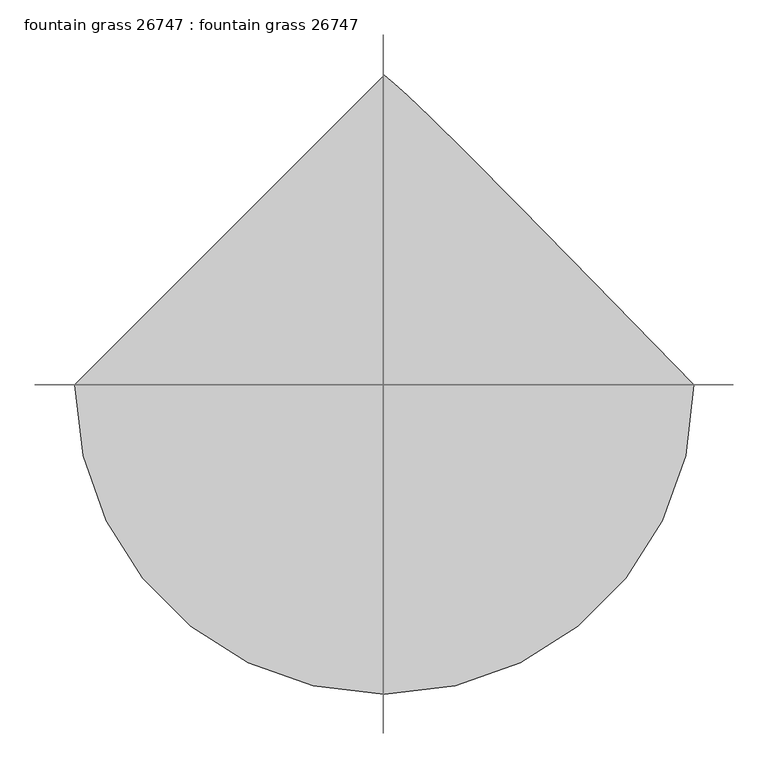
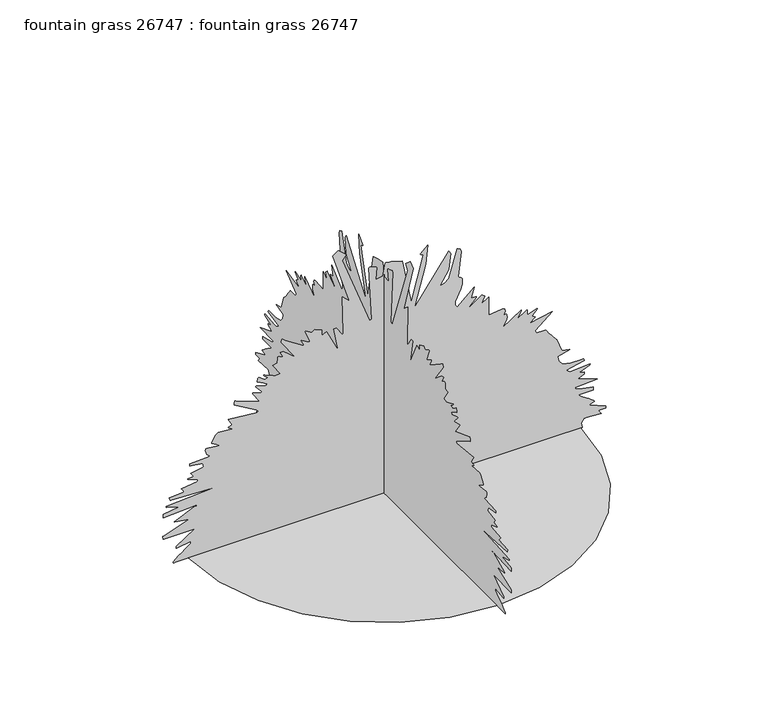
"""IFC4 building model written with IfcOpenShell, lengths in millimetres: proxy geometry, fountain grass 26747 : fountain grass 26747."""

import ifcopenshell
import ifcopenshell.guid

model = None  # the IFC model being written
_history = None  # IfcOwnerHistory: only IFC2X3 demands one
_inside = {}  # id of a spatial element -> (the spatial element, [elements in it])
_under = {}  # id of a project, library or spatial element -> (it, [spatial elements below it])
_declared = {}  # id of a project -> (the project, [libraries it declares])
_typed = {}  # id of a type object -> (the type object, [elements of that type])
_made_of = {}  # id of a material, layer set ... -> (it, [elements and type objects made of it])


def new_model(schema):
    """Start an empty IFC model of exactly this schema.

    Asked for "IFC4X3", IfcOpenShell would pick the latest addendum, in which some entities
    have other attributes; the version numbers below select the first issue.
    IFC2X3 requires an IfcOwnerHistory on every rooted entity: one is made here for all.
    """
    global model, _history
    if schema == "IFC4X3":
        model = ifcopenshell.file(schema_version=(4, 3, 0, 0))
    else:
        model = ifcopenshell.file(schema=schema)
    _inside.clear()
    _under.clear()
    _declared.clear()
    _typed.clear()
    _made_of.clear()
    _history = None
    if model.schema == "IFC2X3":
        org = make("IfcOrganization", Name="unknown")
        user = make(
            "IfcPersonAndOrganization",
            ThePerson=make("IfcPerson", FamilyName="unknown"),
            TheOrganization=org,
        )
        app = make(
            "IfcApplication",
            ApplicationDeveloper=org,
            Version="unknown",
            ApplicationFullName="unknown",
            ApplicationIdentifier="unknown",
        )
        _history = make(
            "IfcOwnerHistory",
            OwningUser=user,
            OwningApplication=app,
            ChangeAction="ADDED",
            CreationDate=0,
        )
    return model


def make(cls, **values):
    """One entity of the class cls with the attributes given. An attribute that is None is left unset."""
    return model.create_entity(
        cls, **{name: value for name, value in values.items() if value is not None}
    )


def rooted(cls, **values):
    """An entity with a GlobalId (a new one), such as an element, a storey or a relation."""
    return make(cls, GlobalId=ifcopenshell.guid.new(), OwnerHistory=_history, **values)


def si_unit(unit_type, name, prefix=None):
    """IfcSIUnit, for example si_unit("LENGTHUNIT", "METRE", prefix="MILLI")."""
    return make("IfcSIUnit", UnitType=unit_type, Prefix=prefix, Name=name)


def assignment(units):
    """IfcUnitAssignment: the units of a project."""
    return None if units is None else make("IfcUnitAssignment", Units=units)


def point(xyz):
    """IfcCartesianPoint."""
    return None if xyz is None else make("IfcCartesianPoint", Coordinates=xyz)


def direction(xyz):
    """IfcDirection."""
    return None if xyz is None else make("IfcDirection", DirectionRatios=xyz)


def frame(location, z_axis=None, x_axis=None):
    """IfcAxis2Placement3D, a coordinate frame: its origin and axes. An axis left out is left unset."""
    return make(
        "IfcAxis2Placement3D",
        Location=point(location),
        Axis=direction(z_axis),
        RefDirection=direction(x_axis),
    )


def origin():
    """The frame at (0, 0, 0) with its axes left unset."""
    return frame((0.0, 0.0, 0.0))


def place(relative_to, where):
    """IfcLocalPlacement: puts the frame where relative to a parent placement (None: the world)."""
    return make(
        "IfcLocalPlacement", PlacementRelTo=relative_to, RelativePlacement=where
    )


def context(
    kind, dimensions, precision=None, world=None, true_north=None, identifier=None
):
    """IfcGeometricRepresentationContext, for example the 3D "Model" context."""
    return make(
        "IfcGeometricRepresentationContext",
        ContextIdentifier=identifier,
        ContextType=kind,
        CoordinateSpaceDimension=dimensions,
        Precision=precision,
        WorldCoordinateSystem=world,
        TrueNorth=true_north,
    )


def project(units=None, contexts=None):
    """IfcProject with its units and contexts."""
    return rooted(
        "IfcProject",
        Name="project",
        RepresentationContexts=contexts,
        UnitsInContext=assignment(units),
    )


def spatial(cls, under=None, at=None, **own):
    """A site, building, storey or space (cls), placed at a placement, below another one or the project."""
    s = rooted(cls, ObjectPlacement=at, **own)
    if under is not None:
        _under.setdefault(under.id(), (under, []))[1].append(s)
    return s


def point_list(points):
    """IfcCartesianPointList2D or 3D."""
    cls = (
        "IfcCartesianPointList2D" if len(points[0]) == 2 else "IfcCartesianPointList3D"
    )
    return make(cls, CoordList=points)


def triangles(points, corners, closed=None, point_numbers=None):
    """IfcTriangulatedFaceSet: each triangle names its three corners, points numbered from 1."""
    return make(
        "IfcTriangulatedFaceSet",
        Coordinates=point_list(points),
        Closed=closed,
        CoordIndex=corners,
        PnIndex=point_numbers,
    )


def shape(context_of_items, identifier, shape_type, items):
    """IfcShapeRepresentation: the items that make up one representation, for example the "Body"."""
    return make(
        "IfcShapeRepresentation",
        ContextOfItems=context_of_items,
        RepresentationIdentifier=identifier,
        RepresentationType=shape_type,
        Items=items,
    )


def source(mapping_origin, context_of_items, identifier, shape_type, items):
    """IfcRepresentationMap: a shape defined once, which mapped items show again and again."""
    return make(
        "IfcRepresentationMap",
        MappingOrigin=mapping_origin,
        MappedRepresentation=shape(context_of_items, identifier, shape_type, items),
    )


def transform(
    local_origin,
    x_axis=None,
    y_axis=None,
    z_axis=None,
    scale=None,
    scale2=None,
    scale3=None,
    uniform=True,
):
    """IfcCartesianTransformationOperator3D, or its non-uniform kind. x_axis, y_axis, z_axis: its Axis1, 2, 3."""
    if uniform:
        return make(
            "IfcCartesianTransformationOperator3D",
            Axis1=direction(x_axis),
            Axis2=direction(y_axis),
            LocalOrigin=point(local_origin),
            Scale=scale,
            Axis3=direction(z_axis),
        )
    return make(
        "IfcCartesianTransformationOperator3DnonUniform",
        Axis1=direction(x_axis),
        Axis2=direction(y_axis),
        LocalOrigin=point(local_origin),
        Scale=scale,
        Axis3=direction(z_axis),
        Scale2=scale2,
        Scale3=scale3,
    )


def mapped(mapping_source, mapping_target):
    """IfcMappedItem: shows the shape of a source again, moved by a transform."""
    return make(
        "IfcMappedItem", MappingSource=mapping_source, MappingTarget=mapping_target
    )


def made_of(thing, what):
    """Note that an element or type object is made of a material, layer set ...; save() writes the relation."""
    if what is not None:
        _made_of.setdefault(what.id(), (what, []))[1].append(thing)
    return thing


def element(
    cls,
    number,
    at=None,
    inside=None,
    cuts=None,
    type_object=None,
    material=None,
    context=None,
    identifier="Body",
    shape_type=None,
    held_by="IfcProductDefinitionShape",
    body=None,
    shapes=None,
    **own,
):
    """One element of the class cls, such as IfcWall. Its Tag is "e" and its number.

    at: its placement. inside: the storey or other place that contains it. cuts: it is an
    opening in that element (IfcRelVoidsElement). A single representation is given by context,
    identifier, shape_type and body (its items); several are given by shapes. held_by: the class
    of the entity that holds the representations. save() writes the other relations.
    """
    e = rooted(cls, Tag="e%d" % number, ObjectPlacement=at, **own)
    if body is not None:
        shapes = [shape(context, identifier, shape_type, body)]
    if shapes is not None:
        e.Representation = make(held_by, Representations=shapes)
    if inside is not None:
        _inside.setdefault(inside.id(), (inside, []))[1].append(e)
    if cuts is not None:
        rooted(
            "IfcRelVoidsElement", RelatingBuildingElement=cuts, RelatedOpeningElement=e
        )
    if type_object is not None:
        _typed.setdefault(type_object.id(), (type_object, []))[1].append(e)
    return made_of(e, material)


def aggregate(whole, parts):
    """IfcRelAggregates: a whole, such as a stair, and the parts it consists of."""
    return rooted("IfcRelAggregates", RelatingObject=whole, RelatedObjects=parts)


def save(model, path):
    """Write the relations noted so far, then the file.

    IfcRelAggregates (storeys below a building ...), IfcRelContainedInSpatialStructure (elements
    in a storey), IfcRelDefinesByType, IfcRelAssociatesMaterial and IfcRelDeclares: one each for
    every whole, place, type object, material and project.
    """
    for whole, parts in _under.values():
        aggregate(whole, parts)
    for where, things in _inside.values():
        rooted(
            "IfcRelContainedInSpatialStructure",
            RelatedElements=things,
            RelatingStructure=where,
        )
    for kind, things in _typed.values():
        rooted("IfcRelDefinesByType", RelatedObjects=things, RelatingType=kind)
    for what, things in _made_of.values():
        rooted("IfcRelAssociatesMaterial", RelatedObjects=things, RelatingMaterial=what)
    for by, libraries in _declared.values():
        rooted("IfcRelDeclares", RelatingContext=by, RelatedDefinitions=libraries)
    model.write(path)


def fountain_grass_26747_fountain_grass_26747_87ae7408(model_context):
    return source(origin(), model_context, "Body", "Tessellation", [
        triangles([(-987.0455658, 0.0, 0.0001807), (-960.952173, -226.1654466, 0.0001807), (-886.6343983, -433.862035, 0.0001807), (-770.0484913, -617.1406734, 0.0001807), (-617.1406734, -770.0484913, 0.0001807), (-433.862035, -886.6343983, 0.0001807), (-226.1654466, -960.952173, 0.0001807), (4.31e-05, -987.0455658, 0.0001807), (226.1657009, -960.952173, 0.0001807), (433.862035, -886.6343983, 0.0001807), (617.1406734, -770.0484913, 0.0001807), (770.0484913, -617.1406734, 0.0001807), (886.6343983, -433.862035, 0.0001807), (960.952173, -226.1654466, 0.0001807), (987.0455658, 8.63e-05, 0.0001807), (666.2769184, 329.0287173, 0.0001807), (428.4772619, 571.2784656, 0.0001807), (259.8137924, 741.2118793, 0.0001807), (146.4631077, 853.2918114, 0.0001807), (74.5956602, 921.9810053, 0.0001807), (30.3837036, 961.7446392, 0.0001807), (-0.0001294, 987.0455658, 0.0001807), (-192.732222, -8.8e-06, 1335.7745705), (-213.2038286, -7.2e-06, 1310.1839813), (-75.0206025, 1.47e-05, 941.6939009), (-74.0421966, 1.47e-05, 941.9784039), (-72.5994794, 1.47e-05, 942.7098999), (-70.8743122, 1.46e-05, 943.7080948), (-69.0480519, 1.45e-05, 944.7977812), (-67.3038361, 1.45e-05, 945.7985195), (-65.8220043, 1.44e-05, 946.5300882), (-64.7846675, 1.44e-05, 946.8119751), (-80.1384406, -2.1e-06, 1223.1789722), (-79.3512975, -2.1e-06, 1223.3695129), (-78.4244554, -2.1e-06, 1223.8850338), (-77.4526488, -2.1e-06, 1224.6394936), (-76.5311389, -2.2e-06, 1225.5436535), (-75.2199908, -2.3e-06, 1227.4587982), (-75.0206025, -2.4e-06, 1228.2971191), (-39.1952093, -1.4e-06, 1212.9427511), (-44.3130519, 2.2e-06, 1151.5281858), (-8.4877319, 1.9e-06, 1156.6462601), (4.7327266, -1.8e-06, 1221.0427654), (6.8660195, -2.1e-06, 1223.1789722), (43.5436857, -1.6e-06, 1215.9958351), (88.7523407, -8e-07, 1202.7066027), (134.8136643, 1.32e-05, 967.2843447), (196.2285203, -5e-07, 1197.5909992), (183.550624, -1e-06, 1203.2526449), (181.3428736, -1.1e-06, 1205.4269308), (180.8747518, -1.1e-06, 1207.8246769), (216.700145, -3.3e-06, 1243.6512691), (206.4644507, 2.5e-06, 1146.4100389), (150.1674419, 1.53e-05, 931.4576797), (324.1773419, -3.2e-06, 1172.2011972), (334.4109833, -2.3e-06, 1156.8469019), (324.1773419, 2.6e-06, 1074.959967), (278.1144741, 6.8e-06, 1003.3091806), (303.186799, 6.4e-06, 1010.2737991), (322.3333048, 5.3e-06, 1028.8183794), (365.1195376, -3.2e-06, 1172.2011972), (380.7405318, -2.8e-06, 1165.3635332), (386.8136713, -1.8e-06, 1149.1050053), (371.0377447, 5.8e-06, 1020.4236883), (372.5033166, 6e-06, 1017.0835579), (375.3150999, 6.2e-06, 1014.6375589), (378.9295232, 6.3e-06, 1012.7299719), (382.8157322, 6.4e-06, 1011.0028244), (386.4301191, 6.5e-06, 1009.0952374), (389.2419024, 6.6e-06, 1006.6492384), (390.7100178, 6.8e-06, 1003.3091806), (390.8116467, 8.5e-06, 974.9780611), (383.7479064, 1e-05, 950.4898756), (355.0433722, 1.34e-05, 892.7557543), (354.7944775, 1.44e-05, 876.299128), (365.1195376, 1.54e-05, 860.0101513), (452.1246194, 1.08e-05, 936.7764685), (436.7703604, 1.39e-05, 885.5980516), (437.4358357, 1.38e-05, 884.2035873), (460.8495229, 1.41e-05, 882.1284233), (462.3608042, 1.42e-05, 880.4799774), (460.8800079, 1.46e-05, 876.8274387), (425.4318083, 1.61e-05, 841.6561117), (426.5341393, 1.66e-05, 839.537709), (430.7911832, 1.6e-05, 840.3353348), (487.9487409, 1.42e-05, 880.4799774), (489.1120783, 1.43e-05, 881.361319), (491.0831062, 1.43e-05, 880.6425402), (503.3030362, 1.48e-05, 870.2437563), (487.9487409, 1.69e-05, 834.4196348), (523.7754058, 1.54e-05, 860.0101513), (523.7754058, 2.12e-05, 762.7688484), (593.7116893, 2.08e-05, 769.8782982), (604.2222033, 2.1e-05, 765.8219324), (607.2778307, 2.16e-05, 755.5679798), (600.5443027, 2.27e-05, 737.1784046), (610.7779804, 2.27e-05, 737.1784046), (611.8422323, 2.27e-05, 736.5230667), (614.1129513, 2.29e-05, 734.0897123), (616.2186367, 2.32e-05, 729.1722799), (616.7773962, 2.37e-05, 721.0722656), (614.4152584, 2.44e-05, 709.086006), (595.4261922, 2.67e-05, 670.6456924), (687.546841, 2.3e-05, 732.0602577), (687.8186268, 2.35e-05, 728.1842588), (667.0770149, 2.55e-05, 691.118062), (716.0887762, 2.38e-05, 722.0933516), (718.2554317, 2.36e-05, 721.8266527), (719.3450455, 2.39e-05, 719.0986942), (717.5061316, 2.5e-05, 697.6534916), (718.2554317, 2.51e-05, 696.2361362), (720.4347319, 2.49e-05, 695.6976517), (766.5382404, 2.45e-05, 712.7029364), (769.4337759, 2.42e-05, 711.5904316), (768.6387663, 2.44e-05, 709.4415802), (744.2522461, 2.59e-05, 683.2440514), (743.8433321, 2.61e-05, 680.8819136), (759.1976274, 2.67e-05, 670.6456924), (728.4915802, 2.82e-05, 645.0577194), (845.0825741, 2.67e-05, 669.6881201), (759.1976274, 3.09e-05, 598.994906), (764.3157017, 3.19e-05, 583.6431541), (810.3760443, 3.19e-05, 583.6431541), (812.6900019, 3.21e-05, 579.4623047), (818.8519804, 3.26e-05, 570.8923699), (827.7013676, 3.33e-05, 559.353176), (838.0696301, 3.41e-05, 546.269636), (848.7985537, 3.49e-05, 533.064192), (858.7223665, 3.56e-05, 521.1643006), (866.6750788, 3.61e-05, 511.9923677), (892.2629791, 4.01e-05, 445.4596919), (933.2077909, 4.07e-05, 435.2234708), (871.793153, 4.16e-05, 419.8692118), (876.9112272, 4.31e-05, 394.2787316), (879.8754358, 4.33e-05, 391.6269676), (882.8904408, 4.35e-05, 388.2919604), (885.7733316, 4.37e-05, 384.6267408), (888.3361839, 4.39e-05, 380.9920063), (890.3960873, 4.41e-05, 377.7407876), (891.7651897, 4.43e-05, 375.2261882), (892.2629791, 4.44e-05, 373.8088692), (895.890156, 4.44e-05, 372.7801892), (938.3258652, 4.5e-05, 363.5726844), (999.7404305, 4.5e-05, 363.5726844), (1000.5278824, 4.5e-05, 362.5440044), (1001.4549334, 4.51e-05, 361.080976), (1002.425223, 4.52e-05, 359.3588428), (1003.3472597, 4.53e-05, 357.5503776), (1004.1219217, 4.54e-05, 355.8282443), (1004.6578629, 4.55e-05, 354.3652159), (1004.8585773, 4.56e-05, 353.3364996), (912.7354214, 4.68e-05, 332.86413), (913.6015022, 4.69e-05, 331.6373154), (915.8976557, 4.7e-05, 329.6383458), (919.1819029, 4.71e-05, 327.1415142), (923.0020912, 4.73e-05, 324.4110123), (926.9110823, 4.75e-05, 321.7160823), (930.4620283, 4.76e-05, 319.3259302), (933.2077909, 4.77e-05, 317.5123781), (949.6695042, 4.77e-05, 318.6757155), (1032.0797356, 4.76e-05, 324.6954789), (1035.5645519, 4.74e-05, 322.6279452), (1033.032221, 4.76e-05, 319.7526484), (979.2680609, 4.89e-05, 297.0400085), (1004.8585773, 4.92e-05, 291.9219162), (1004.8585773, 4.99e-05, 281.6857132), (975.3971489, 5.07e-05, 267.6446189), (974.1499866, 5.08e-05, 266.331436), (1071.3912169, 5.29e-05, 230.5068058), (958.7956913, 5.32e-05, 225.3889678), (958.7956913, 5.35e-05, 220.2708572), (979.2680609, 5.41e-05, 210.0351811), (1050.9188473, 5.5e-05, 194.6814126), (1050.9188473, 5.6e-05, 179.327626), (974.1499866, 5.6e-05, 179.327626), (978.767728, 5.62e-05, 175.5818881), (990.6523224, 5.67e-05, 167.0838239), (1006.8625975, 5.74e-05, 155.6789786), (1024.4520761, 5.81e-05, 143.2134423), (1051.9830992, 5.94e-05, 122.4842661), (1056.0369942, 5.96e-05, 117.9127791), (1055.1428627, 5.97e-05, 116.2480642), (1031.9527084, 6.02e-05, 108.5996212), (1030.4464777, 6.02e-05, 107.6770939), (1112.3334852, 6.24e-05, 71.8517007), (1112.3334852, 6.3e-05, 61.6157658), (1076.5093637, 6.3e-05, 61.6157658), (1088.8461107, 6.4e-05, 43.7974311), (1091.8611156, 6.42e-05, 41.1441501), (1004.8585773, 6.39e-05, 46.2622425), (989.504282, 6.51e-05, 25.7906269), (994.6223562, 6.66e-05, 0.2009925), (-1062.775609, 7.09e-05, 6.89e-05), (-1062.775609, 7.05e-05, 5.1179681), (-1049.4888474, 6.99e-05, 15.7529118), (-1033.944084, 6.92e-05, 27.9602914), (-1017.6728388, 6.84e-05, 40.5703616), (-1002.191589, 6.77e-05, 52.4138656), (-989.0343979, 6.71e-05, 62.3213777), (-979.7176701, 6.67e-05, 69.1234924), (-975.7730707, 6.66e-05, 71.6507864), (-975.7730707, 6.6e-05, 81.8864716), (-1047.4213137, 6.66e-05, 71.6507864), (-1047.4213137, 6.6e-05, 81.8864716), (-955.3006285, 6.23e-05, 143.3013185), (-1113.9564966, 6.23e-05, 143.3013185), (-1114.0479881, 6.22e-05, 144.6553964), (-1114.2638906, 6.21e-05, 147.0447673), (-1114.5102419, 6.19e-05, 150.0158069), (-1114.6931522, 6.17e-05, 153.1156177), (-1114.7261444, 6.16e-05, 155.891066), (-1114.5102419, 6.14e-05, 157.8885276), (-1113.9564966, 6.14e-05, 158.6551051), (-986.0066757, 5.87e-05, 204.7161744), (-1054.7643974, 5.81e-05, 213.3275311), (-1057.6574621, 5.8e-05, 214.9521049), (-955.3006285, 5.53e-05, 261.0126836), (-945.06448, 5.53e-05, 261.0126836), (-945.06448, 5.5e-05, 266.130776), (-1113.9564966, 5.56e-05, 255.8945912), (-1113.9564966, 5.44e-05, 276.3669608), (-1032.0695618, 5.38e-05, 286.6031456), (-1098.6022739, 5.26e-05, 307.0755152), (-1098.6022739, 5.22e-05, 312.1910823), (-852.941324, 5.13e-05, 327.5453776), (-1078.1298317, 5.07e-05, 337.7815624), (-1082.9660191, 4.99e-05, 351.3121319), (-1083.2479786, 4.98e-05, 353.1358578), (-1006.4790453, 4.95e-05, 358.253932), (-1021.1679016, 4.84e-05, 377.3064754), (-1021.8333406, 4.83e-05, 378.7237945), (-939.9464058, 4.77e-05, 388.9599792), (-939.9464058, 4.71e-05, 399.196164), (-983.6648129, 4.62e-05, 414.4208888), (-989.0952953, 4.6e-05, 417.5603411), (-991.1248226, 4.58e-05, 419.6685336), (-960.4187754, 4.55e-05, 424.7866442), (-975.1050156, 4.44e-05, 443.8391513), (-975.7730707, 4.43e-05, 445.2590137), (-909.2403585, 4.37e-05, 455.4926551), (-914.3558893, 4.25e-05, 475.965061), (-980.8911449, 4.19e-05, 486.2012458), (-980.8911449, 4.13e-05, 496.4374306), (-878.5317678, 4.1e-05, 501.5555048), (-879.1134184, 4.09e-05, 503.3716003), (-888.6028828, 4.02e-05, 513.6840159), (-893.8860632, 4e-05, 516.9098001), (-900.7211838, 3.88e-05, 540.5851356), (-900.558621, 3.85e-05, 544.4840255), (-899.0041374, 3.82e-05, 547.6158474), (-894.7090508, 3.84e-05, 548.9721963), (-839.7257063, 3.85e-05, 543.0539892), (-832.4714979, 3.85e-05, 542.4977368), (-834.0945093, 3.85e-05, 545.8555987), (-865.9461262, 3.72e-05, 565.5888419), (-868.2956194, 3.7e-05, 568.088217), (-868.4048424, 3.65e-05, 572.164894), (-848.5039495, 3.46e-05, 604.96896), (-842.4562082, 3.44e-05, 611.1792641), (-837.5895721, 3.42e-05, 614.1485596), (-765.9387857, 3.46e-05, 609.030449), (-780.5183464, 3.41e-05, 617.4352776), (-785.6364206, 3.37e-05, 622.5609821), (-786.4086119, 3.36e-05, 624.384708), (-767.3586119, 3.34e-05, 628.6646067), (-765.9387857, 3.33e-05, 629.5027822), (-786.4086119, 3.12e-05, 665.3269037), (-637.9889648, 3.21e-05, 649.9752245), (-637.7984241, 3.21e-05, 650.9530718), (-637.2828306, 3.2e-05, 652.395789), (-636.5284435, 3.19e-05, 654.1204657), (-635.6242109, 3.18e-05, 655.946735), (-634.6564648, 3.17e-05, 657.6916866), (-633.7090662, 3.16e-05, 659.1725555), (-632.8733614, 3.15e-05, 660.2088295), (-755.7025646, 2.72e-05, 731.8596159), (-755.710195, 2.71e-05, 734.6180958), (-755.6593987, 2.69e-05, 738.1944036), (-755.4384092, 2.67e-05, 742.1339161), (-754.9329895, 2.65e-05, 745.9743793), (-754.0313004, 2.63e-05, 749.26117), (-752.6190319, 2.61e-05, 751.5344324), (-750.5844904, 2.6e-05, 752.3319855), (-627.7552872, 2.88e-05, 706.2717155), (-663.6860882, 2.56e-05, 759.6675116), (-663.5794086, 2.54e-05, 762.5682066), (-660.4755283, 2.56e-05, 763.5054314), (-620.4934484, 2.58e-05, 751.3083561), (-617.5191387, 2.6e-05, 752.3319855), (-618.27854, 2.56e-05, 755.4434961), (-647.6638103, 2.37e-05, 790.1982788), (-648.2251133, 2.36e-05, 793.2742538), (-645.0653498, 2.38e-05, 794.1149729), (-597.0467328, 2.45e-05, 777.9225019), (-596.4675894, 2.44e-05, 778.9130665), (-595.0452198, 2.43e-05, 780.3888485), (-593.2570295, 2.42e-05, 782.1490608), (-591.5755551, 2.41e-05, 784.0032354), (-590.4782747, 2.4e-05, 785.7507305), (-590.4376522, 2.39e-05, 787.201078), (-591.9286222, 2.39e-05, 788.1586504), (-637.9889648, 2.24e-05, 813.7466234), (-639.6145197, 2.21e-05, 815.2045286), (-640.0666723, 2.19e-05, 818.265243), (-638.3851616, 2.15e-05, 826.5253492), (-636.7163681, 2.14e-05, 830.3861601), (-634.8012234, 2.12e-05, 833.1724726), (-632.8733614, 2.11e-05, 834.218993), (-630.4730719, 2.12e-05, 834.2443548), (-602.164807, 2.24e-05, 813.7466234), (-586.810548, 2.2e-05, 818.8646976), (-606.0256179, 2.11e-05, 834.9200403), (-607.7909171, 2.1e-05, 837.6987951), (-607.2829176, 2.08e-05, 839.3370672), (-603.6684943, 2.09e-05, 838.9128925), (-561.8702826, 2.2e-05, 820.0915123), (-550.9864265, 2.24e-05, 813.7466234), (-525.3959464, 2.2e-05, 818.8646976), (-559.8662261, 1.89e-05, 871.7906096), (-561.2226113, 1.87e-05, 875.1611887), (-540.7502054, 1.84e-05, 880.2793356), (-537.9714506, 1.73e-05, 906.7536644), (-536.9859366, 1.7e-05, 909.870262), (-535.6321312, 1.66e-05, 910.9878536), (-533.2191244, 1.68e-05, 912.2654646), (-529.3558064, 1.69e-05, 911.5212513), (-510.0416511, 1.72e-05, 900.7517052), (-525.3959464, 1.53e-05, 931.4576797), (-510.0416511, 1.53e-05, 931.4576797), (-448.6270494, 1.84e-05, 880.2793356), (-520.2778358, 1.23e-05, 982.63864), (-520.4962818, 1.22e-05, 984.7163475), (-516.051277, 1.16e-05, 996.9642191), (-515.2257823, 1.15e-05, 998.3459661), (-515.1597616, 1.14e-05, 997.9903919), (-498.3728866, 1.21e-05, 985.7882298), (-408.0734565, 1.55e-05, 927.9093498), (-402.5667432, 1.56e-05, 926.342149), (-417.4790597, 1.45e-05, 951.9148613), (-418.5687098, 1.42e-05, 955.282897), (-417.9210385, 1.38e-05, 957.0481962), (-415.5080317, 1.41e-05, 957.1853245), (-380.6389392, 1.48e-05, 937.1701944), (-376.976263, 1.5e-05, 936.5758266), (-376.9203798, 1.43e-05, 940.7439589), (-397.9032924, 1.21e-05, 994.048336), (-397.4486326, 1.14e-05, 997.9903919), (-395.0686543, 1.16e-05, 998.5085289), (-366.1584277, 1.23e-05, 982.382115), (-351.3883264, 1.17e-05, 992.8748611), (-315.5616614, 1.26e-05, 977.5205658), (-315.5616614, 1.44e-05, 946.8119751), (-294.1621864, 1.4e-05, 958.3587994), (-291.1294318, 1.39e-05, 958.6407589), (-289.9737247, 1.38e-05, 957.0481962), (-233.6754533, 2.08e-05, 839.3370672), (-254.1470598, 1.35e-05, 962.1662704), (-243.9113837, 1.35e-05, 962.1662704), (-213.2038286, 1.62e-05, 916.1059278), (-211.0877513, 1.6e-05, 916.598703), (-209.5368286, 1.59e-05, 917.6680418), (-208.4642015, 1.57e-05, 919.1971636), (-207.7817031, 1.56e-05, 921.0716858), (-207.4032379, 1.54e-05, 923.1722116), (-207.2399121, 1.53e-05, 925.3845766), (-207.2046126, 1.52e-05, 927.5918547), (-213.2038286, 4.4e-06, 1115.7040644), (-210.5383663, 4.8e-06, 1115.4424524), (-179.2496511, 6.1e-06, 1087.4745375), (-177.3786897, 6.2e-06, 1084.9954737), (-259.2651522, -9.7e-06, 1351.1262497), (-233.6754533, -1.09e-05, 1371.5986919), (-3.3699163, -189.3624059, 1335.7745705), (-3.3699163, -209.8340125, 1310.1839813), (-3.3699163, -71.6505366, 941.6939009), (-3.3699163, -70.6721261, 941.9784039), (-3.3699163, -69.2296633, 942.7098999), (-3.3699163, -67.5042417, 943.7080948), (-3.3699163, -65.6782403, 944.7977812), (-3.3699163, -63.93402, 945.7985195), (-3.3699163, -62.4519338, 946.5300882), (-3.3699163, -61.4148514, 946.8119751), (-3.3699163, -76.7683792, 1223.1789722), (-3.3699163, -75.9812316, 1223.3695129), (-3.3699163, -75.054385, 1223.8850338), (-3.3699163, -74.0828373, 1224.6394936), (-3.3699163, -73.161073, 1225.5436535), (-3.3699163, -71.8499249, 1227.4587982), (-3.3699163, -71.6505366, 1228.2971191), (-3.3699163, -35.8251411, 1212.9427511), (-3.3699163, -40.9429814, 1151.5281858), (-3.3699163, -5.1177648, 1156.6462601), (-3.3699163, 8.1026934, 1221.0427654), (-3.3699163, 10.2359611, 1223.1789722), (-3.3699163, 46.9137516, 1215.9958351), (-3.3699163, 92.122402, 1202.7066027), (-3.3699163, 138.1834804, 967.2843447), (-3.3699163, 199.5985907, 1197.5909992), (-3.3699163, 186.9206945, 1203.2526449), (-3.3699163, 184.7129259, 1205.4269308), (-3.3699163, 184.244804, 1207.8246769), (-3.3699163, 220.0701972, 1243.6512691), (-3.3699163, 209.8342668, 1146.4100389), (-3.3699163, 153.5372671, 931.4576797), (-3.3699163, 327.5453776, 1172.2011972), (-3.3699163, 337.7815624, 1156.8469019), (-3.3699163, 327.5453776, 1074.959967), (-3.3699163, 281.4850532, 1003.3091806), (-3.3699163, 306.5573782, 1010.2737991), (-3.3699163, 325.7038839, 1028.8183794), (-3.3699163, 368.4901168, 1172.2011972), (-3.3699163, 384.1085675, 1165.3635332), (-3.3699163, 390.1842505, 1149.1050053), (-3.3699163, 374.4057804, 1020.4236883), (-3.3699163, 375.8738957, 1017.0835579), (-3.3699163, 378.6856791, 1014.6375589), (-3.3699163, 382.3001023, 1012.7299719), (-3.3699163, 386.1863113, 1011.0028244), (-3.3699163, 389.8006983, 1009.0952374), (-3.3699163, 392.6124816, 1006.6492384), (-3.3699163, 394.0780535, 1003.3091806), (-3.3699163, 394.1796824, 974.9780611), (-3.3699163, 387.1184855, 950.4898756), (-3.3699163, 358.4139513, 892.7557543), (-3.3699163, 358.1650566, 876.299128), (-3.3699163, 368.4901168, 860.0101513), (-3.3699163, 455.4926551, 936.7764685), (-3.3699163, 440.1409032, 885.5980516), (-3.3699163, 440.8038714, 884.2035873), (-3.3699163, 464.2175586, 882.1284233), (-3.3699163, 465.7288399, 880.4799774), (-3.3699163, 464.2505871, 876.8274387), (-3.3699163, 428.8023874, 841.6561117), (-3.3699163, 429.9047184, 839.537709), (-3.3699163, 434.1617623, 840.3353348), (-3.3699163, 491.31932, 880.4799774), (-3.3699163, 492.480114, 881.361319), (-3.3699163, 494.4536854, 880.6425402), (-3.3699163, 506.6736154, 870.2437563), (-3.3699163, 491.31932, 834.4196348), (-3.3699163, 527.1434415, 860.0101513), (-3.3699163, 527.1434415, 762.7688484), (-3.3699163, 597.079725, 769.8782982), (-3.3699163, 607.5927824, 765.8219324), (-3.3699163, 610.6458664, 755.5679798), (-3.3699163, 603.9123384, 737.1784046), (-3.3699163, 614.1485596, 737.1784046), (-3.3699163, 615.2128115, 736.5230667), (-3.3699163, 617.4835304, 734.0897123), (-3.3699163, 619.5866724, 729.1722799), (-3.3699163, 620.1479753, 721.0722656), (-3.3699163, 617.7858376, 709.086006), (-3.3699163, 598.7942279, 670.6456924), (-3.3699163, 690.9174202, 732.0602577), (-3.3699163, 691.1866625, 728.1842588), (-3.3699163, 670.4450506, 691.118062), (-3.3699163, 719.4568119, 722.0933516), (-3.3699163, 721.6260109, 721.8266527), (-3.3699163, 722.7156246, 719.0986942), (-3.3699163, 720.8767107, 697.6534916), (-3.3699163, 721.6260109, 696.2361362), (-3.3699163, 723.805311, 695.6976517), (-3.3699163, 769.9062761, 712.7029364), (-3.3699163, 772.804355, 711.5904316), (-3.3699163, 772.0093454, 709.4415802), (-3.3699163, 747.6202818, 683.2440514), (-3.3699163, 747.2139112, 680.8819136), (-3.3699163, 762.5682066, 670.6456924), (-3.3699163, 731.8596159, 645.0577194), (-3.3699163, 848.4531532, 669.6881201), (-3.3699163, 762.5682066, 598.994906), (-3.3699163, 767.6862808, 583.6431541), (-3.3699163, 813.7466234, 583.6431541), (-3.3699163, 816.0605083, 579.4623047), (-3.3699163, 822.2225595, 570.8923699), (-3.3699163, 831.0694033, 559.353176), (-3.3699163, 841.4402092, 546.269636), (-3.3699163, 852.1691328, 533.064192), (-3.3699163, 862.0904022, 521.1643006), (-3.3699163, 870.0431145, 511.9923677), (-3.3699163, 895.6335583, 445.4596919), (-3.3699163, 936.5758266, 435.2234708), (-3.3699163, 875.1611887, 419.8692118), (-3.3699163, 880.2793356, 394.2787316), (-3.3699163, 883.246015, 391.6269676), (-3.3699163, 886.2610199, 388.289417), (-3.3699163, 889.1439108, 384.6267408), (-3.3699163, 891.7067631, 380.9920063), (-3.3699163, 893.764123, 377.7407876), (-3.3699163, 895.1357689, 375.2261882), (-3.3699163, 895.6335583, 373.8088692), (-3.3699163, 899.2607351, 372.7801892), (-3.3699163, 941.6939009, 363.5726844), (-3.3699163, 1003.1084661, 363.5726844), (-3.3699163, 1003.8959181, 362.5440044), (-3.3699163, 1004.8229691, 361.080976), (-3.3699163, 1005.7958021, 359.3588428), (-3.3699163, 1006.7178389, 357.5503776), (-3.3699163, 1007.4925009, 355.8282443), (-3.3699163, 1008.028442, 354.3652159), (-3.3699163, 1008.226613, 353.3364996), (-3.3699163, 916.1059278, 332.86413), (-3.3699163, 916.9695379, 331.6373154), (-3.3699163, 919.2682348, 329.6383458), (-3.3699163, 922.5499386, 327.1415142), (-3.3699163, 926.3701269, 324.4110123), (-3.3699163, 930.279118, 321.7160823), (-3.3699163, 933.8326075, 319.3259302), (-3.3699163, 936.5758266, 317.5098347), (-3.3699163, 953.0400833, 318.6757155), (-3.3699163, 1035.4503147, 324.6954789), (-3.3699163, 1038.9351311, 322.6279452), (-3.3699163, 1036.4028002, 319.7501049), (-3.3699163, 982.63864, 297.0400085), (-3.3699163, 1008.226613, 291.9219162), (-3.3699163, 1008.226613, 281.6857132), (-3.3699163, 978.767728, 267.6446189), (-3.3699163, 977.5205658, 266.331436), (-3.3699163, 1074.7592525, 230.5068058), (-3.3699163, 962.1662704, 225.3887135), (-3.3699163, 962.1662704, 220.2708572), (-3.3699163, 982.63864, 210.0351811), (-3.3699163, 1054.2894264, 194.6814126), (-3.3699163, 1054.2894264, 179.327626), (-3.3699163, 977.5205658, 179.327626), (-3.3699163, 982.1357637, 175.5818881), (-3.3699163, 994.0229015, 167.0835696), (-3.3699163, 1010.2331766, 155.6787243), (-3.3699163, 1027.8226553, 143.2131879), (-3.3699163, 1055.3536783, 122.4842661), (-3.3699163, 1059.4075733, 117.9127791), (-3.3699163, 1058.5134418, 116.2478099), (-3.3699163, 1035.3207441, 108.5993669), (-3.3699163, 1033.8170568, 107.6768396), (-3.3699163, 1115.7040644, 71.8517007), (-3.3699163, 1115.7040644, 61.6157658), (-3.3699163, 1079.8773994, 61.6157658), (-3.3699163, 1092.2166899, 43.7971768), (-3.3699163, 1095.2316948, 41.1441501), (-3.3699163, 1008.226613, 46.2619882), (-3.3699163, 992.8748611, 25.7903726), (-3.3699163, 997.9929354, 0.2009237), (-3.3699163, -1059.4050299, 0.0), (-3.3699163, -1059.4050299, 5.117917), (-3.3699163, -1046.1182682, 15.7528607), (-3.3699163, -1030.5760483, 27.9600371), (-3.3699163, -1014.3022596, 40.5701072), (-3.3699163, -998.8235533, 52.4138656), (-3.3699163, -985.6638187, 62.3213777), (-3.3699163, -976.3496344, 69.1234924), (-3.3699163, -972.4024916, 71.6507864), (-3.3699163, -972.4024916, 81.8864716), (-3.3699163, -1044.053278, 71.6507864), (-3.3699163, -1044.053278, 81.8864716), (-3.3699163, -951.930122, 143.3013185), (-3.3699163, -1110.5859175, 143.3013185), (-3.3699163, -1110.677409, 144.6553964), (-3.3699163, -1110.8933115, 147.0447673), (-3.3699163, -1111.1396627, 150.0158069), (-3.3699163, -1111.3251165, 153.1156177), (-3.3699163, -1111.3555653, 155.891066), (-3.3699163, -1111.1396627, 157.8885276), (-3.3699163, -1110.5859175, 158.6551051), (-3.3699163, -982.63864, 204.7161744), (-3.3699163, -1051.3938183, 213.3275311), (-3.3699163, -1054.2894264, 214.9521049), (-3.3699163, -951.930122, 261.0126836), (-3.3699163, -941.6939009, 261.0126836), (-3.3699163, -941.6939009, 266.130776), (-3.3699163, -1110.5859175, 255.8945912), (-3.3699163, -1110.5859175, 276.3669608), (-3.3699163, -1028.6989826, 286.6031456), (-3.3699163, -1095.2316948, 307.0755152), (-3.3699163, -1095.2316948, 312.1910823), (-3.3699163, -849.5732883, 327.5453776), (-3.3699163, -1074.7592525, 337.7815624), (-3.3699163, -1079.5954399, 351.3121319), (-3.3699163, -1079.8773994, 353.1358578), (-3.3699163, -1003.1084661, 358.253932), (-3.3699163, -1017.7973225, 377.3064754), (-3.3699163, -1018.4627615, 378.7237945), (-3.3699163, -936.5758266, 388.9599792), (-3.3699163, -936.5758266, 399.196164), (-3.3699163, -980.2942337, 414.4208888), (-3.3699163, -985.7272596, 417.5603411), (-3.3699163, -987.7567869, 419.6685336), (-3.3699163, -957.0481962, 424.7866442), (-3.3699163, -971.7369799, 443.8391513), (-3.3699163, -972.4024916, 445.2590137), (-3.3699163, -905.8697794, 455.4926551), (-3.3699163, -910.9878536, 475.965061), (-3.3699163, -977.5205658, 486.2012458), (-3.3699163, -977.5205658, 496.4374306), (-3.3699163, -875.1611887, 501.5555048), (-3.3699163, -875.7428392, 503.3690932), (-3.3699163, -885.2348471, 513.6814725), (-3.3699163, -890.515484, 516.9098001), (-3.3699163, -897.3506046, 540.5851356), (-3.3699163, -897.1880419, 544.4840255), (-3.3699163, -895.6335583, 547.6158474), (-3.3699163, -891.3384716, 548.9721963), (-3.3699163, -836.3576706, 543.0539892), (-3.3699163, -829.1009188, 542.4977368), (-3.3699163, -830.7239302, 545.8555987), (-3.3699163, -862.5780905, 565.5888419), (-3.3699163, -864.9250402, 568.088217), (-3.3699163, -865.0368067, 572.1623506), (-3.3699163, -845.1333704, 604.96896), (-3.3699163, -839.0856291, 611.1792641), (-3.3699163, -834.218993, 614.1485596), (-3.3699163, -762.5682066, 609.030449), (-3.3699163, -777.1477673, 617.4352776), (-3.3699163, -782.2658415, 622.5609821), (-3.3699163, -783.0405762, 624.384708), (-3.3699163, -763.9880327, 628.6646067), (-3.3699163, -762.5682066, 629.5027822), (-3.3699163, -783.0405762, 665.3269037), (-3.3699163, -634.6209291, 649.9752245), (-3.3699163, -634.427845, 650.9530718), (-3.3699163, -633.9122515, 652.395789), (-3.3699163, -633.1604078, 654.1204657), (-3.3699163, -632.2561752, 655.946735), (-3.3699163, -631.2858856, 657.6916866), (-3.3699163, -630.3410305, 659.1725555), (-3.3699163, -629.5027822, 660.2088295), (-3.3699163, -752.3319855, 731.8596159), (-3.3699163, -752.3396158, 734.6180958), (-3.3699163, -752.291363, 738.1944036), (-3.3699163, -752.0703735, 742.1339161), (-3.3699163, -751.5649538, 745.9743793), (-3.3699163, -750.6632647, 749.26117), (-3.3699163, -749.2484528, 751.5344324), (-3.3699163, -747.2139112, 752.3319855), (-3.3699163, -624.384708, 706.2717155), (-3.3699163, -660.315509, 759.6675116), (-3.3699163, -660.2088295, 762.5682066), (-3.3699163, -657.1049492, 763.5054314), (-3.3699163, -617.1228693, 751.3083561), (-3.3699163, -614.1485596, 752.3319855), (-3.3699163, -614.9079609, 755.4434961), (-3.3699163, -644.2932312, 790.1982788), (-3.3699163, -644.8570776, 793.2742538), (-3.3699163, -641.6947706, 794.1149729), (-3.3699163, -593.6761537, 777.9225019), (-3.3699163, -593.0970102, 778.9130665), (-3.3699163, -591.6771841, 780.3888485), (-3.3699163, -589.8864867, 782.1490608), (-3.3699163, -588.2075194, 784.0032354), (-3.3699163, -587.1076956, 785.7507305), (-3.3699163, -587.0670731, 787.201078), (-3.3699163, -588.5580431, 788.1586504), (-3.3699163, -634.6209291, 813.7466234), (-3.3699163, -636.2439405, 815.2045286), (-3.3699163, -636.6960932, 818.265243), (-3.3699163, -635.0171259, 826.5253492), (-3.3699163, -633.3458616, 830.3861601), (-3.3699163, -631.4306442, 833.1724726), (-3.3699163, -629.5027822, 834.218993), (-3.3699163, -627.1050362, 834.2443548), (-3.3699163, -598.7942279, 813.7466234), (-3.3699163, -583.4399689, 818.8646976), (-3.3699163, -602.6575822, 834.9200403), (-3.3699163, -604.420338, 837.6987951), (-3.3699163, -603.9123384, 839.3370672), (-3.3699163, -600.2979152, 838.9128925), (-3.3699163, -558.5022469, 820.0915123), (-3.3699163, -547.6158474, 813.7466234), (-3.3699163, -522.0253673, 818.8646976), (-3.3699163, -556.495647, 871.7906096), (-3.3699163, -557.8520322, 875.1611887), (-3.3699163, -537.3796263, 880.2793356), (-3.3699163, -534.6008715, 906.7536644), (-3.3699163, -533.6153575, 909.870262), (-3.3699163, -532.261552, 910.9878536), (-3.3699163, -529.8510887, 912.2654646), (-3.3699163, -525.9877707, 911.5212513), (-3.3699163, -506.6736154, 900.7517052), (-3.3699163, -522.0253673, 931.4576797), (-3.3699163, -506.6736154, 931.4576797), (-3.3699163, -445.2564703, 880.2793356), (-3.3699163, -516.9072567, 982.63864), (-3.3699163, -517.1282461, 984.7163475), (-3.3699163, -512.6832413, 996.9642191), (-3.3699163, -511.8552032, 998.3459661), (-3.3699163, -511.7891825, 997.9929354), (-3.3699163, -495.0023074, 985.7882298), (-3.3699163, -404.7028773, 927.9093498), (-3.3699163, -399.196164, 926.342149), (-3.3699163, -414.111024, 951.9148613), (-3.3699163, -415.1981306, 955.282897), (-3.3699163, -414.5504594, 957.0481962), (-3.3699163, -412.1374526, 957.1853245), (-3.3699163, -377.2709035, 937.1701944), (-3.3699163, -373.6056839, 936.5758266), (-3.3699163, -373.5523441, 940.7439589), (-3.3699163, -394.5327132, 994.048336), (-3.3699163, -394.0780535, 997.9929354), (-3.3699163, -391.6980752, 998.5085289), (-3.3699163, -362.790392, 982.382115), (-3.3699163, -348.0177472, 992.8748611), (-3.3699163, -312.1910823, 977.5205658), (-3.3699163, -312.1910823, 946.8119751), (-3.3699163, -290.7916072, 958.3587994), (-3.3699163, -287.7613961, 958.6407589), (-3.3699163, -286.6031456, 957.0481962), (-3.3699163, -230.3056372, 839.3370672), (-3.3699163, -250.7772437, 962.1662704), (-3.3699163, -240.5415676, 962.1662704), (-3.3699163, -209.8340125, 916.1059278), (-3.3699163, -207.7176991, 916.598703), (-3.3699163, -206.1670306, 917.6680418), (-3.3699163, -205.094131, 919.1971636), (-3.3699163, -204.411887, 921.0716858), (-3.3699163, -204.0334218, 923.1722116), (-3.3699163, -203.8698416, 925.3845766), (-3.3699163, -203.8347965, 927.5918547), (-3.3699163, -209.8340125, 1115.7040644), (-3.3699163, -207.1682958, 1115.4424524), (-3.3699163, -175.879835, 1087.4745375), (-3.3699163, -174.0086193, 1084.9954737), (-3.3699163, -255.8945912, 1351.1262497), (-3.3699163, -230.3056372, 1371.5986919)], [[21, 22, 1], [20, 21, 1], [19, 20, 1], [18, 19, 1], [17, 18, 1], [17, 1, 2], [17, 2, 3], [17, 3, 4], [16, 17, 4], [16, 4, 5], [16, 5, 6], [16, 6, 7], [16, 7, 8], [16, 8, 9], [16, 9, 10], [16, 10, 11], [16, 11, 12], [15, 16, 12], [14, 15, 12], [13, 14, 12], [168, 169, 170], [119, 120, 121], [131, 132, 133], [76, 77, 78], [188, 189, 190], [333, 334, 335], [215, 216, 217], [266, 267, 268], [90, 91, 92], [235, 236, 237], [234, 235, 237], [214, 215, 217], [103, 104, 105], [103, 105, 106], [327, 328, 329], [233, 234, 237], [54, 55, 56], [54, 56, 57], [54, 57, 58], [230, 231, 232], [117, 118, 119], [238, 239, 240], [229, 230, 232], [60, 61, 62], [60, 62, 63], [191, 192, 193], [161, 162, 163], [38, 39, 40], [356, 357, 358], [356, 358, 359], [237, 238, 240], [202, 203, 204], [202, 204, 205], [187, 188, 190], [319, 320, 321], [366, 367, 368], [366, 368, 369], [366, 369, 370], [227, 228, 229], [219, 220, 221], [219, 221, 222], [191, 193, 194], [191, 194, 195], [191, 195, 196], [191, 196, 197], [191, 197, 198], [191, 198, 199], [191, 199, 200], [191, 200, 201], [185, 186, 187], [184, 185, 187], [184, 187, 190], [173, 174, 175], [172, 173, 175], [113, 114, 115], [191, 201, 202], [191, 202, 205], [226, 227, 229], [225, 226, 229], [225, 229, 232], [150, 151, 152], [149, 150, 152], [148, 149, 152], [147, 148, 152], [146, 147, 152], [145, 146, 152], [144, 145, 152], [143, 144, 152], [372, 23, 24], [371, 372, 24], [370, 371, 24], [370, 24, 25], [366, 370, 25], [242, 243, 244], [241, 242, 244], [223, 224, 225], [222, 223, 225], [219, 222, 225], [205, 206, 207], [291, 292, 293], [333, 335, 336], [205, 207, 208], [76, 78, 79], [205, 208, 209], [205, 209, 210], [205, 210, 211], [205, 211, 212], [205, 212, 213], [205, 213, 214], [332, 333, 336], [331, 332, 336], [330, 331, 336], [330, 336, 337], [365, 366, 25], [37, 38, 40], [60, 63, 64], [262, 263, 264], [32, 33, 34], [313, 314, 315], [312, 313, 315], [311, 312, 315], [364, 365, 25], [164, 165, 166], [160, 161, 163], [160, 163, 164], [318, 319, 321], [37, 40, 41], [36, 37, 41], [35, 36, 41], [34, 35, 41], [32, 34, 41], [32, 41, 42], [112, 113, 115], [112, 115, 116], [171, 172, 175], [363, 364, 25], [262, 264, 265], [261, 262, 265], [346, 347, 348], [346, 348, 349], [285, 286, 287], [290, 291, 293], [290, 293, 294], [180, 181, 182], [233, 237, 240], [350, 351, 352], [340, 341, 342], [339, 340, 342], [338, 339, 342], [338, 342, 343], [284, 285, 287], [284, 287, 288], [179, 180, 182], [179, 182, 183], [179, 183, 184], [330, 337, 338], [80, 81, 82], [79, 80, 82], [76, 79, 82], [76, 82, 83], [261, 265, 266], [261, 266, 268], [356, 359, 360], [214, 217, 218], [205, 214, 218], [191, 205, 218], [191, 218, 219], [191, 219, 225], [190, 191, 225], [184, 190, 225], [179, 184, 225], [178, 179, 225], [177, 178, 225], [176, 177, 225], [175, 176, 225], [171, 175, 225], [170, 171, 225], [168, 170, 225], [107, 108, 109], [106, 107, 109], [106, 109, 110], [362, 363, 25], [122, 123, 124], [142, 143, 152], [112, 116, 117], [112, 117, 119], [111, 112, 119], [130, 131, 133], [275, 276, 277], [275, 277, 278], [275, 278, 279], [275, 279, 280], [275, 280, 281], [275, 281, 282], [275, 282, 283], [275, 283, 284], [353, 354, 355], [349, 350, 352], [346, 349, 352], [345, 346, 352], [344, 345, 352], [86, 87, 88], [289, 290, 294], [60, 64, 65], [59, 60, 65], [50, 51, 52], [49, 50, 52], [48, 49, 52], [48, 52, 53], [47, 48, 53], [47, 53, 54], [284, 288, 289], [164, 166, 167], [160, 164, 167], [160, 167, 168], [159, 160, 168], [159, 168, 225], [158, 159, 225], [157, 158, 225], [156, 157, 225], [155, 156, 225], [154, 155, 225], [153, 154, 225], [152, 153, 225], [142, 152, 225], [141, 142, 225], [140, 141, 225], [139, 140, 225], [138, 139, 225], [137, 138, 225], [136, 137, 225], [135, 136, 225], [134, 135, 225], [133, 134, 225], [130, 133, 225], [129, 130, 225], [128, 129, 225], [127, 128, 225], [126, 127, 225], [125, 126, 225], [124, 125, 225], [122, 124, 225], [121, 122, 225], [119, 121, 225], [111, 119, 225], [110, 111, 225], [225, 232, 233], [225, 233, 240], [43, 44, 45], [93, 94, 95], [93, 95, 96], [92, 93, 96], [311, 315, 316], [42, 43, 45], [42, 45, 46], [32, 42, 46], [32, 46, 47], [32, 47, 54], [353, 355, 356], [352, 353, 356], [344, 352, 356], [59, 65, 66], [249, 250, 251], [248, 249, 251], [247, 248, 251], [246, 247, 251], [245, 246, 251], [245, 251, 252], [244, 245, 252], [244, 252, 253], [327, 329, 330], [76, 83, 84], [361, 362, 25], [240, 241, 244], [225, 240, 244], [225, 244, 253], [255, 256, 257], [254, 255, 257], [254, 257, 258], [254, 258, 259], [254, 259, 260], [254, 260, 261], [253, 254, 261], [302, 303, 304], [225, 253, 261], [225, 261, 268], [356, 360, 361], [356, 361, 25], [86, 88, 89], [85, 86, 89], [85, 89, 90], [85, 90, 92], [84, 85, 92], [324, 325, 326], [301, 302, 304], [301, 304, 305], [301, 305, 306], [301, 306, 307], [301, 307, 308], [301, 308, 309], [301, 309, 310], [301, 310, 311], [301, 311, 316], [300, 301, 316], [300, 316, 317], [299, 300, 317], [338, 343, 344], [338, 344, 356], [330, 338, 356], [323, 324, 326], [322, 323, 326], [322, 326, 327], [321, 322, 327], [318, 321, 327], [318, 327, 330], [318, 330, 356], [96, 97, 98], [96, 98, 99], [96, 99, 100], [96, 100, 101], [96, 101, 102], [92, 96, 102], [92, 102, 103], [59, 66, 67], [284, 289, 294], [59, 67, 68], [59, 68, 69], [59, 69, 70], [59, 70, 71], [59, 71, 72], [59, 72, 73], [58, 59, 73], [54, 58, 73], [54, 73, 74], [54, 74, 75], [54, 75, 76], [299, 317, 318], [298, 299, 318], [298, 318, 356], [297, 298, 356], [296, 297, 356], [295, 296, 356], [294, 295, 356], [284, 294, 356], [275, 284, 356], [274, 275, 356], [273, 274, 356], [272, 273, 356], [271, 272, 356], [270, 271, 356], [269, 270, 356], [268, 269, 356], [225, 268, 356], [76, 84, 92], [76, 92, 103], [54, 76, 103], [32, 54, 103], [31, 32, 103], [30, 31, 103], [29, 30, 103], [28, 29, 103], [27, 28, 103], [26, 27, 103], [25, 26, 103], [356, 25, 103], [225, 356, 103], [110, 225, 103], [110, 103, 106], [518, 519, 520], [469, 470, 471], [481, 482, 483], [426, 427, 428], [538, 539, 540], [683, 684, 685], [565, 566, 567], [616, 617, 618], [440, 441, 442], [585, 586, 587], [584, 585, 587], [564, 565, 567], [453, 454, 455], [453, 455, 456], [677, 678, 679], [583, 584, 587], [404, 405, 406], [404, 406, 407], [404, 407, 408], [580, 581, 582], [467, 468, 469], [588, 589, 590], [579, 580, 582], [410, 411, 412], [410, 412, 413], [541, 542, 543], [511, 512, 513], [388, 389, 390], [706, 707, 708], [706, 708, 709], [587, 588, 590], [552, 553, 554], [552, 554, 555], [537, 538, 540], [669, 670, 671], [716, 717, 718], [716, 718, 719], [716, 719, 720], [577, 578, 579], [569, 570, 571], [569, 571, 572], [541, 543, 544], [541, 544, 545], [541, 545, 546], [541, 546, 547], [541, 547, 548], [541, 548, 549], [541, 549, 550], [541, 550, 551], [535, 536, 537], [534, 535, 537], [534, 537, 540], [523, 524, 525], [522, 523, 525], [463, 464, 465], [541, 551, 552], [541, 552, 555], [576, 577, 579], [575, 576, 579], [575, 579, 582], [500, 501, 502], [499, 500, 502], [498, 499, 502], [497, 498, 502], [496, 497, 502], [495, 496, 502], [494, 495, 502], [493, 494, 502], [722, 373, 374], [721, 722, 374], [720, 721, 374], [720, 374, 375], [716, 720, 375], [592, 593, 594], [591, 592, 594], [573, 574, 575], [572, 573, 575], [569, 572, 575], [555, 556, 557], [641, 642, 643], [683, 685, 686], [555, 557, 558], [426, 428, 429], [555, 558, 559], [555, 559, 560], [555, 560, 561], [555, 561, 562], [555, 562, 563], [555, 563, 564], [682, 683, 686], [681, 682, 686], [680, 681, 686], [680, 686, 687], [715, 716, 375], [387, 388, 390], [410, 413, 414], [612, 613, 614], [382, 383, 384], [663, 664, 665], [662, 663, 665], [661, 662, 665], [714, 715, 375], [514, 515, 516], [510, 511, 513], [510, 513, 514], [668, 669, 671], [387, 390, 391], [386, 387, 391], [385, 386, 391], [384, 385, 391], [382, 384, 391], [382, 391, 392], [462, 463, 465], [462, 465, 466], [521, 522, 525], [713, 714, 375], [612, 614, 615], [611, 612, 615], [696, 697, 698], [696, 698, 699], [635, 636, 637], [640, 641, 643], [640, 643, 644], [530, 531, 532], [583, 587, 590], [700, 701, 702], [690, 691, 692], [689, 690, 692], [688, 689, 692], [688, 692, 693], [634, 635, 637], [634, 637, 638], [529, 530, 532], [529, 532, 533], [529, 533, 534], [680, 687, 688], [430, 431, 432], [429, 430, 432], [426, 429, 432], [426, 432, 433], [611, 615, 616], [611, 616, 618], [706, 709, 710], [564, 567, 568], [555, 564, 568], [541, 555, 568], [541, 568, 569], [541, 569, 575], [540, 541, 575], [534, 540, 575], [529, 534, 575], [528, 529, 575], [527, 528, 575], [526, 527, 575], [525, 526, 575], [521, 525, 575], [520, 521, 575], [518, 520, 575], [457, 458, 459], [456, 457, 459], [456, 459, 460], [712, 713, 375], [472, 473, 474], [492, 493, 502], [462, 466, 467], [462, 467, 469], [461, 462, 469], [480, 481, 483], [625, 626, 627], [625, 627, 628], [625, 628, 629], [625, 629, 630], [625, 630, 631], [625, 631, 632], [625, 632, 633], [625, 633, 634], [703, 704, 705], [699, 700, 702], [696, 699, 702], [695, 696, 702], [694, 695, 702], [436, 437, 438], [639, 640, 644], [410, 414, 415], [409, 410, 415], [400, 401, 402], [399, 400, 402], [398, 399, 402], [398, 402, 403], [397, 398, 403], [397, 403, 404], [634, 638, 639], [514, 516, 517], [510, 514, 517], [510, 517, 518], [509, 510, 518], [509, 518, 575], [508, 509, 575], [507, 508, 575], [506, 507, 575], [505, 506, 575], [504, 505, 575], [503, 504, 575], [502, 503, 575], [492, 502, 575], [491, 492, 575], [490, 491, 575], [489, 490, 575], [488, 489, 575], [487, 488, 575], [486, 487, 575], [485, 486, 575], [484, 485, 575], [483, 484, 575], [480, 483, 575], [479, 480, 575], [478, 479, 575], [477, 478, 575], [476, 477, 575], [475, 476, 575], [474, 475, 575], [472, 474, 575], [471, 472, 575], [469, 471, 575], [461, 469, 575], [460, 461, 575], [575, 582, 583], [575, 583, 590], [393, 394, 395], [443, 444, 445], [443, 445, 446], [442, 443, 446], [661, 665, 666], [392, 393, 395], [392, 395, 396], [382, 392, 396], [382, 396, 397], [382, 397, 404], [703, 705, 706], [702, 703, 706], [694, 702, 706], [409, 415, 416], [599, 600, 601], [598, 599, 601], [597, 598, 601], [596, 597, 601], [595, 596, 601], [595, 601, 602], [594, 595, 602], [594, 602, 603], [677, 679, 680], [426, 433, 434], [711, 712, 375], [590, 591, 594], [575, 590, 594], [575, 594, 603], [605, 606, 607], [604, 605, 607], [604, 607, 608], [604, 608, 609], [604, 609, 610], [604, 610, 611], [603, 604, 611], [652, 653, 654], [575, 603, 611], [575, 611, 618], [706, 710, 711], [706, 711, 375], [436, 438, 439], [435, 436, 439], [435, 439, 440], [435, 440, 442], [434, 435, 442], [674, 675, 676], [651, 652, 654], [651, 654, 655], [651, 655, 656], [651, 656, 657], [651, 657, 658], [651, 658, 659], [651, 659, 660], [651, 660, 661], [651, 661, 666], [650, 651, 666], [650, 666, 667], [649, 650, 667], [688, 693, 694], [688, 694, 706], [680, 688, 706], [673, 674, 676], [672, 673, 676], [672, 676, 677], [671, 672, 677], [668, 671, 677], [668, 677, 680], [668, 680, 706], [446, 447, 448], [446, 448, 449], [446, 449, 450], [446, 450, 451], [446, 451, 452], [442, 446, 452], [442, 452, 453], [409, 416, 417], [634, 639, 644], [409, 417, 418], [409, 418, 419], [409, 419, 420], [409, 420, 421], [409, 421, 422], [409, 422, 423], [408, 409, 423], [404, 408, 423], [404, 423, 424], [404, 424, 425], [404, 425, 426], [649, 667, 668], [648, 649, 668], [648, 668, 706], [647, 648, 706], [646, 647, 706], [645, 646, 706], [644, 645, 706], [634, 644, 706], [625, 634, 706], [624, 625, 706], [623, 624, 706], [622, 623, 706], [621, 622, 706], [620, 621, 706], [619, 620, 706], [618, 619, 706], [575, 618, 706], [426, 434, 442], [426, 442, 453], [404, 426, 453], [382, 404, 453], [381, 382, 453], [380, 381, 453], [379, 380, 453], [378, 379, 453], [377, 378, 453], [376, 377, 453], [375, 376, 453], [706, 375, 453], [575, 706, 453], [460, 575, 453], [460, 453, 456]], closed=False),
    ])


if __name__ == "__main__":
    model = new_model("IFC4")
    model_context = context("Model", 3, world=origin())
    ifc_project = project(units=[si_unit("LENGTHUNIT", "METRE", prefix="MILLI")], contexts=[model_context])
    site = spatial("IfcSite", under=ifc_project)
    building = spatial("IfcBuilding", under=site)
    placement = place(None, origin())
    fountain_grass_26747_fountain_grass_26747_shape = fountain_grass_26747_fountain_grass_26747_87ae7408(model_context)
    element("IfcBuildingElementProxy", 1, Name="fountain grass 26747 : fountain grass 26747", ObjectType="fountain grass 26747 : fountain grass 26747", at=placement, inside=building, context=model_context, shape_type="MappedRepresentation", body=[
        mapped(fountain_grass_26747_fountain_grass_26747_shape, transform((0.0, 0.0, 0.0), x_axis=(1.0, 0.0, 0.0), y_axis=(0.0, 1.0, 0.0), z_axis=(0.0, 0.0, 1.0))),
    ])
    save(model, "model.ifc")

# Revit data of these elements
# Type "fountain grass 26747 : fountain grass 26747"
#   built-in parameter 1005195 = "RPC-16-FXGG-QKFX-PG74-4000-ST1L-LVER-AU"
#   Height = 0
